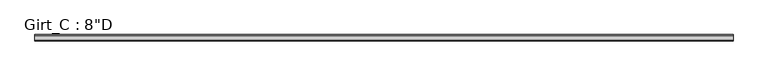
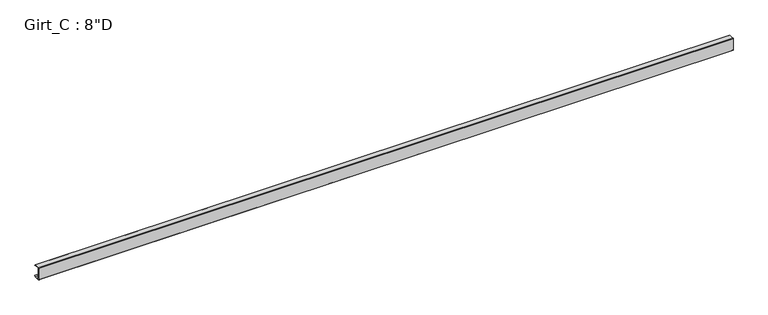
"""IFC4 building model written with IfcOpenShell, lengths in millimetres: beam geometry."""

import ifcopenshell
import ifcopenshell.guid

model = None  # the IFC model being written
_history = None  # IfcOwnerHistory: only IFC2X3 demands one
_inside = {}  # id of a spatial element -> (the spatial element, [elements in it])
_under = {}  # id of a project, library or spatial element -> (it, [spatial elements below it])
_declared = {}  # id of a project -> (the project, [libraries it declares])
_typed = {}  # id of a type object -> (the type object, [elements of that type])
_made_of = {}  # id of a material, layer set ... -> (it, [elements and type objects made of it])


def new_model(schema):
    """Start an empty IFC model of exactly this schema.

    Asked for "IFC4X3", IfcOpenShell would pick the latest addendum, in which some entities
    have other attributes; the version numbers below select the first issue.
    IFC2X3 requires an IfcOwnerHistory on every rooted entity: one is made here for all.
    """
    global model, _history
    if schema == "IFC4X3":
        model = ifcopenshell.file(schema_version=(4, 3, 0, 0))
    else:
        model = ifcopenshell.file(schema=schema)
    _inside.clear()
    _under.clear()
    _declared.clear()
    _typed.clear()
    _made_of.clear()
    _history = None
    if model.schema == "IFC2X3":
        org = make("IfcOrganization", Name="unknown")
        user = make(
            "IfcPersonAndOrganization",
            ThePerson=make("IfcPerson", FamilyName="unknown"),
            TheOrganization=org,
        )
        app = make(
            "IfcApplication",
            ApplicationDeveloper=org,
            Version="unknown",
            ApplicationFullName="unknown",
            ApplicationIdentifier="unknown",
        )
        _history = make(
            "IfcOwnerHistory",
            OwningUser=user,
            OwningApplication=app,
            ChangeAction="ADDED",
            CreationDate=0,
        )
    return model


def make(cls, **values):
    """One entity of the class cls with the attributes given. An attribute that is None is left unset."""
    return model.create_entity(
        cls, **{name: value for name, value in values.items() if value is not None}
    )


def rooted(cls, **values):
    """An entity with a GlobalId (a new one), such as an element, a storey or a relation."""
    return make(cls, GlobalId=ifcopenshell.guid.new(), OwnerHistory=_history, **values)


def si_unit(unit_type, name, prefix=None):
    """IfcSIUnit, for example si_unit("LENGTHUNIT", "METRE", prefix="MILLI")."""
    return make("IfcSIUnit", UnitType=unit_type, Prefix=prefix, Name=name)


def assignment(units):
    """IfcUnitAssignment: the units of a project."""
    return None if units is None else make("IfcUnitAssignment", Units=units)


def point(xyz):
    """IfcCartesianPoint."""
    return None if xyz is None else make("IfcCartesianPoint", Coordinates=xyz)


def direction(xyz):
    """IfcDirection."""
    return None if xyz is None else make("IfcDirection", DirectionRatios=xyz)


def frame(location, z_axis=None, x_axis=None):
    """IfcAxis2Placement3D, a coordinate frame: its origin and axes. An axis left out is left unset."""
    return make(
        "IfcAxis2Placement3D",
        Location=point(location),
        Axis=direction(z_axis),
        RefDirection=direction(x_axis),
    )


def frame_2d(location, x_axis=None):
    """IfcAxis2Placement2D, a coordinate frame in the plane: its origin and x axis."""
    return make(
        "IfcAxis2Placement2D", Location=point(location), RefDirection=direction(x_axis)
    )


def origin():
    """The frame at (0, 0, 0) with its axes left unset."""
    return frame((0.0, 0.0, 0.0))


def place(relative_to, where):
    """IfcLocalPlacement: puts the frame where relative to a parent placement (None: the world)."""
    return make(
        "IfcLocalPlacement", PlacementRelTo=relative_to, RelativePlacement=where
    )


def context(
    kind, dimensions, precision=None, world=None, true_north=None, identifier=None
):
    """IfcGeometricRepresentationContext, for example the 3D "Model" context."""
    return make(
        "IfcGeometricRepresentationContext",
        ContextIdentifier=identifier,
        ContextType=kind,
        CoordinateSpaceDimension=dimensions,
        Precision=precision,
        WorldCoordinateSystem=world,
        TrueNorth=true_north,
    )


def project(units=None, contexts=None):
    """IfcProject with its units and contexts."""
    return rooted(
        "IfcProject",
        Name="project",
        RepresentationContexts=contexts,
        UnitsInContext=assignment(units),
    )


def spatial(cls, under=None, at=None, **own):
    """A site, building, storey or space (cls), placed at a placement, below another one or the project."""
    s = rooted(cls, ObjectPlacement=at, **own)
    if under is not None:
        _under.setdefault(under.id(), (under, []))[1].append(s)
    return s


def polyline(points):
    """IfcPolyline through the points."""
    return make("IfcPolyline", Points=[point(p) for p in points])


def circle_curve(where, radius):
    """IfcCircle in the frame where."""
    return make("IfcCircle", Position=where, Radius=radius)


def trimmed(basis, trim1, trim2, sense, master):
    """IfcTrimmedCurve: the piece of a basis curve between two trims."""
    return make(
        "IfcTrimmedCurve",
        BasisCurve=basis,
        Trim1=trim1,
        Trim2=trim2,
        SenseAgreement=sense,
        MasterRepresentation=master,
    )


def segment(curve, same_sense, transition):
    """IfcCompositeCurveSegment."""
    return make(
        "IfcCompositeCurveSegment",
        Transition=transition,
        SameSense=same_sense,
        ParentCurve=curve,
    )


def composite_curve(segments, self_intersect=None):
    """IfcCompositeCurve: segments joined end to end."""
    return make("IfcCompositeCurve", Segments=segments, SelfIntersect=self_intersect)


def outline(outer, holes=None, kind="AREA"):
    """IfcArbitraryClosedProfileDef: a profile drawn as a closed curve; with holes, ...WithVoids."""
    if holes is None:
        return make("IfcArbitraryClosedProfileDef", ProfileType=kind, OuterCurve=outer)
    return make(
        "IfcArbitraryProfileDefWithVoids",
        ProfileType=kind,
        OuterCurve=outer,
        InnerCurves=holes,
    )


def extrude(swept, where, along, depth):
    """IfcExtrudedAreaSolid: the profile swept, set in the frame where, extruded along a direction by depth."""
    return make(
        "IfcExtrudedAreaSolid",
        SweptArea=swept,
        Position=where,
        ExtrudedDirection=direction(along),
        Depth=depth,
    )


def shape(context_of_items, identifier, shape_type, items):
    """IfcShapeRepresentation: the items that make up one representation, for example the "Body"."""
    return make(
        "IfcShapeRepresentation",
        ContextOfItems=context_of_items,
        RepresentationIdentifier=identifier,
        RepresentationType=shape_type,
        Items=items,
    )


def source(mapping_origin, context_of_items, identifier, shape_type, items):
    """IfcRepresentationMap: a shape defined once, which mapped items show again and again."""
    return make(
        "IfcRepresentationMap",
        MappingOrigin=mapping_origin,
        MappedRepresentation=shape(context_of_items, identifier, shape_type, items),
    )


def transform(
    local_origin,
    x_axis=None,
    y_axis=None,
    z_axis=None,
    scale=None,
    scale2=None,
    scale3=None,
    uniform=True,
):
    """IfcCartesianTransformationOperator3D, or its non-uniform kind. x_axis, y_axis, z_axis: its Axis1, 2, 3."""
    if uniform:
        return make(
            "IfcCartesianTransformationOperator3D",
            Axis1=direction(x_axis),
            Axis2=direction(y_axis),
            LocalOrigin=point(local_origin),
            Scale=scale,
            Axis3=direction(z_axis),
        )
    return make(
        "IfcCartesianTransformationOperator3DnonUniform",
        Axis1=direction(x_axis),
        Axis2=direction(y_axis),
        LocalOrigin=point(local_origin),
        Scale=scale,
        Axis3=direction(z_axis),
        Scale2=scale2,
        Scale3=scale3,
    )


def mapped(mapping_source, mapping_target):
    """IfcMappedItem: shows the shape of a source again, moved by a transform."""
    return make(
        "IfcMappedItem", MappingSource=mapping_source, MappingTarget=mapping_target
    )


def made_of(thing, what):
    """Note that an element or type object is made of a material, layer set ...; save() writes the relation."""
    if what is not None:
        _made_of.setdefault(what.id(), (what, []))[1].append(thing)
    return thing


def element(
    cls,
    number,
    at=None,
    inside=None,
    cuts=None,
    type_object=None,
    material=None,
    context=None,
    identifier="Body",
    shape_type=None,
    held_by="IfcProductDefinitionShape",
    body=None,
    shapes=None,
    **own,
):
    """One element of the class cls, such as IfcWall. Its Tag is "e" and its number.

    at: its placement. inside: the storey or other place that contains it. cuts: it is an
    opening in that element (IfcRelVoidsElement). A single representation is given by context,
    identifier, shape_type and body (its items); several are given by shapes. held_by: the class
    of the entity that holds the representations. save() writes the other relations.
    """
    e = rooted(cls, Tag="e%d" % number, ObjectPlacement=at, **own)
    if body is not None:
        shapes = [shape(context, identifier, shape_type, body)]
    if shapes is not None:
        e.Representation = make(held_by, Representations=shapes)
    if inside is not None:
        _inside.setdefault(inside.id(), (inside, []))[1].append(e)
    if cuts is not None:
        rooted(
            "IfcRelVoidsElement", RelatingBuildingElement=cuts, RelatedOpeningElement=e
        )
    if type_object is not None:
        _typed.setdefault(type_object.id(), (type_object, []))[1].append(e)
    return made_of(e, material)


def aggregate(whole, parts):
    """IfcRelAggregates: a whole, such as a stair, and the parts it consists of."""
    return rooted("IfcRelAggregates", RelatingObject=whole, RelatedObjects=parts)


def save(model, path):
    """Write the relations noted so far, then the file.

    IfcRelAggregates (storeys below a building ...), IfcRelContainedInSpatialStructure (elements
    in a storey), IfcRelDefinesByType, IfcRelAssociatesMaterial and IfcRelDeclares: one each for
    every whole, place, type object, material and project.
    """
    for whole, parts in _under.values():
        aggregate(whole, parts)
    for where, things in _inside.values():
        rooted(
            "IfcRelContainedInSpatialStructure",
            RelatedElements=things,
            RelatingStructure=where,
        )
    for kind, things in _typed.values():
        rooted("IfcRelDefinesByType", RelatedObjects=things, RelatingType=kind)
    for what, things in _made_of.values():
        rooted("IfcRelAssociatesMaterial", RelatedObjects=things, RelatingMaterial=what)
    for by, libraries in _declared.values():
        rooted("IfcRelDeclares", RelatingContext=by, RelatedDefinitions=libraries)
    model.write(path)


def beam_73cb32fd(model_context):
    return source(origin(), model_context, "Body", "SweptSolid", [
        extrude(outline(composite_curve([segment(polyline([(87.5109375, 101.6), (99.7560415, 87.0068534), (97.6278742, 85.221109), (86.2154765, 98.821875), (3.3005807, 98.821875)]), True, "CONTINUOUS"), segment(trimmed(circle_curve(frame_2d((3.3741066, 96.8381931)), 1.9850441), [point((3.3005807, 98.821875))], [point((1.3890625, 96.8381931))], True, "CARTESIAN"), True, "CONTINUOUS"), segment(polyline([(1.3890625, 96.8381931), (1.3890625, -96.8389339)]), True, "CONTINUOUS"), segment(trimmed(circle_curve(frame_2d((3.3748024, -96.8389339)), 1.9857399), [point((1.3890625, -96.8389339))], [point((3.2694106, -98.821875))], True, "CARTESIAN"), True, "CONTINUOUS"), segment(polyline([(3.2694106, -98.821875), (86.2154765, -98.821875), (97.6510975, -85.1934327), (99.7792647, -86.979177), (87.5109375, -101.6), (3.3734375, -101.6)]), True, "CONTINUOUS"), segment(trimmed(circle_curve(frame_2d((3.3734375, -96.8375)), 4.7625), [point((3.3734375, -101.6))], [point((-1.3890625, -96.8375))], False, "CARTESIAN"), True, "CONTINUOUS"), segment(polyline([(-1.3890625, -96.8375), (-1.3890625, 96.8375)]), True, "CONTINUOUS"), segment(trimmed(circle_curve(frame_2d((3.3734375, 96.8375)), 4.7625), [point((-1.3890625, 96.8375))], [point((3.3734375, 101.6))], False, "CARTESIAN"), True, "CONTINUOUS"), segment(polyline([(3.3734375, 101.6), (87.5109375, 101.6)]), True, "CONTINUOUS")], self_intersect=False)), frame((-5643.4399169, 0.0, 0.0), z_axis=(1.0, 0.0, 0.0), x_axis=(0.0, 1.0, 0.0)), (0.0, 0.0, 1.0), 11286.8798339),
    ])


if __name__ == "__main__":
    model = new_model("IFC4")
    model_context = context("Model", 3, world=origin())
    ifc_project = project(units=[si_unit("LENGTHUNIT", "METRE", prefix="MILLI")], contexts=[model_context])
    site = spatial("IfcSite", under=ifc_project)
    building = spatial("IfcBuilding", under=site)
    placement = place(None, origin())
    beam_shape = beam_73cb32fd(model_context)
    element("IfcBeam", 1, ObjectType="Girt_C : 8\"D", at=placement, inside=building, context=model_context, shape_type="MappedRepresentation", body=[
        mapped(beam_shape, transform((0.0, 0.0, 0.0), x_axis=(1.0, 0.0, 0.0), y_axis=(0.0, 1.0, 0.0), z_axis=(0.0, 0.0, 1.0))),
    ])
    save(model, "model.ifc")

# Revit data of these elements
# Type "Girt_C : 8\"D"
#   half leg = 0' - 1 3/4"
#   Web_Thickness = 0' - 0 7/64"
#   Length [instance default] = 10' - 0"
#   Leg_1 = 0' - 3 1/2"
#   Height = 0' - 8"
#   Structural Material [instance default] = none
# Element 1 (IfcBeam, "Girt_C : 8\"D")
#   Structural Material = GALVANIZED 'CEE' SECTION (8.0x3.5C - SEE STRUCT. DWGS)
#   Materials on its faces: "GALVANIZED 'CEE' SECTION (8.0x3.5C - SEE STRUCT. DWGS)"
# Materials
#   "GALVANIZED 'CEE' SECTION (8.0x3.5C - SEE STRUCT. DWGS)": class "Metal", colour RGB 137 146 153, transparency 0, Description = "Steel, mill finish", Cost = 0
